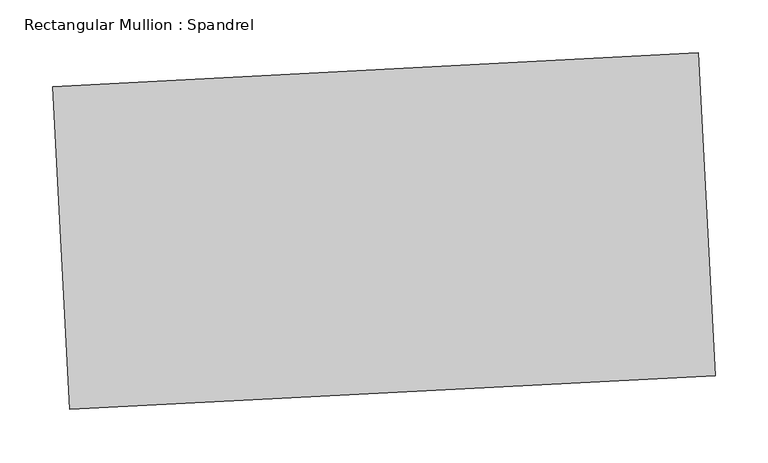
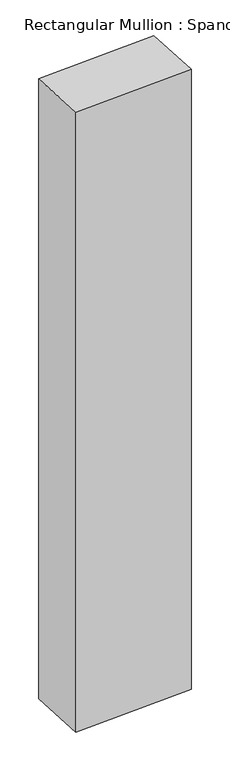
"""IFC4 building model written with IfcOpenShell, lengths in millimetres: member geometry, Rectangular Mullion : Spandrel."""

from ifc_helpers import new_model, si_unit, frame, origin, place, context, project, spatial, polyline, outline, extrude, source, transform, mapped, element, save


def rectangular_mullion_spandrel_3b5c7c06(model_context):
    return source(origin(), model_context, "Body", "SweptSolid", [
        extrude(outline(polyline([(-617.1582819, 136.2391416), (-8.3937175, 168.1431406), (7.5582819, -136.2391416), (-601.2062825, -168.1431406), (-617.1582819, 136.2391416)])), frame((0.0, 0.0, -3352.8), z_axis=(0.0, 0.0, 1.0), x_axis=(1.0, 0.0, 0.0)), (0.0, 0.0, 1.0), 3352.8),
    ])


if __name__ == "__main__":
    model = new_model("IFC4")
    model_context = context("Model", 3, world=origin())
    ifc_project = project(units=[si_unit("LENGTHUNIT", "METRE", prefix="MILLI")], contexts=[model_context])
    site = spatial("IfcSite", under=ifc_project)
    building = spatial("IfcBuilding", under=site)
    placement = place(None, origin())
    rectangular_mullion_spandrel_shape = rectangular_mullion_spandrel_3b5c7c06(model_context)
    element("IfcMember", 1, ObjectType="Rectangular Mullion : Spandrel", at=placement, inside=building, context=model_context, shape_type="MappedRepresentation", body=[
        mapped(rectangular_mullion_spandrel_shape, transform((0.0, 0.0, 0.0), x_axis=(1.0, 0.0, 0.0), y_axis=(0.0, 1.0, 0.0), z_axis=(0.0, 0.0, 1.0))),
    ])
    save(model, "model.ifc")

# Revit data of these elements
# Type "Rectangular Mullion : Spandrel"
#   built-in parameter 1007304 = 1 (stored number, unit not read)
#   built-in parameter 1007301 = 1 (stored number, unit not read)
#   built-in parameter 1007300 = 1 (stored number, unit not read)
# Element 1 (IfcMember, "Rectangular Mullion : Spandrel")
#   Materials on its faces: "Aluminum"
# Materials
#   "Aluminum": class "Metal", colour RGB 247 247 247, transparency 0, Description = "Aluminum 6061", Cost = 0
